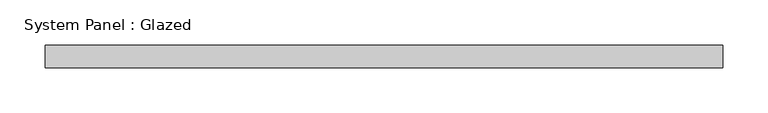
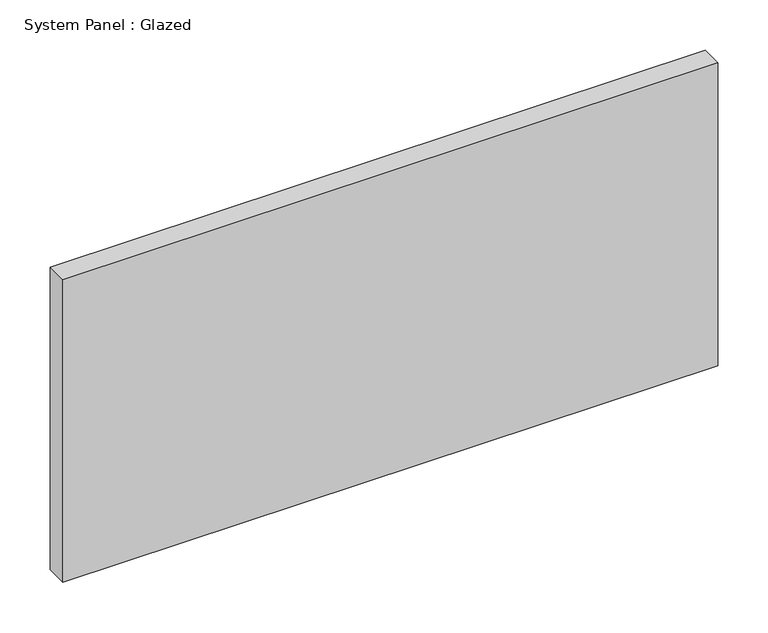
"""IFC4 building model written with IfcOpenShell, lengths in millimetres: plate geometry, System Panel : Glazed."""

from ifc_helpers import new_model, si_unit, origin, origin_with_axes, place, context, project, spatial, polyline, outline, extrude, source, transform, mapped, element, save


def system_panel_glazed_1e0e35d1(model_context):
    return source(origin(), model_context, "Body", "SweptSolid", [
        extrude(outline(polyline([(375.0, 24.5), (-375.0, 24.5), (-375.0, 49.5), (375.0, 49.5), (375.0, 24.5)])), origin_with_axes(), (0.0, 0.0, 1.0), 366.6666667),
    ])


if __name__ == "__main__":
    model = new_model("IFC4")
    model_context = context("Model", 3, world=origin())
    ifc_project = project(units=[si_unit("LENGTHUNIT", "METRE", prefix="MILLI")], contexts=[model_context])
    site = spatial("IfcSite", under=ifc_project)
    building = spatial("IfcBuilding", under=site)
    placement = place(None, origin())
    system_panel_glazed_shape = system_panel_glazed_1e0e35d1(model_context)
    element("IfcPlate", 1, ObjectType="System Panel : Glazed", at=placement, inside=building, context=model_context, shape_type="MappedRepresentation", body=[
        mapped(system_panel_glazed_shape, transform((0.0, 0.0, 0.0), x_axis=(1.0, 0.0, 0.0), y_axis=(0.0, 1.0, 0.0), z_axis=(0.0, 0.0, 1.0))),
    ])
    save(model, "model.ifc")

# Revit data of these elements
# Element 1 (IfcPlate, "System Panel : Glazed")
#   Materials on its faces: "Glass"
# Materials
#   "Glass": class "Glass", colour RGB 218 227 224, transparency 0.85, Description = "Soda Lime Glass", Cost = 0
